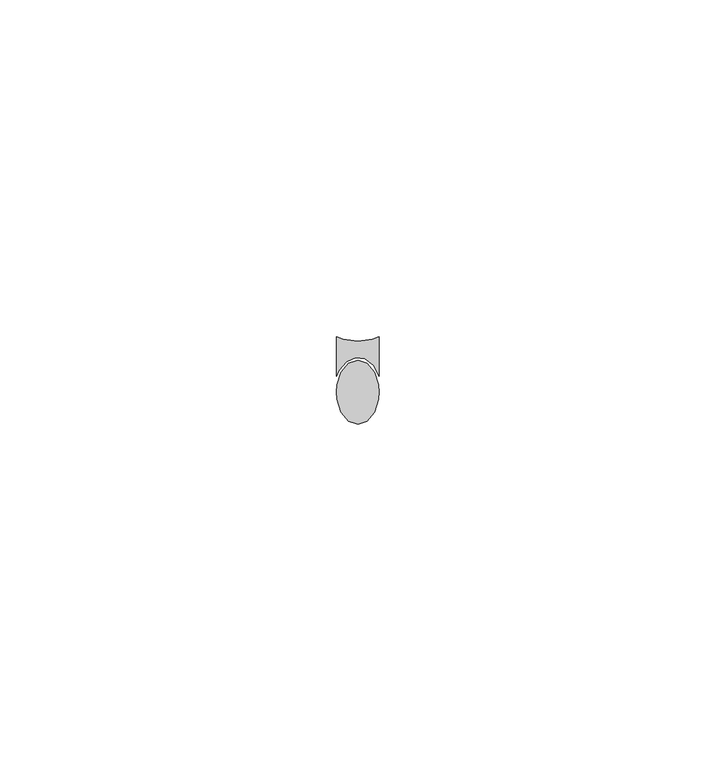
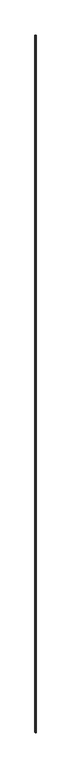
"""IFC4 building model written with IfcOpenShell, lengths in millimetres: proxy geometry, Generic Models 11:Generic Models 1:306267:Generic Models 1:306267 : Generic Models 11:Generic Models 1:306267:300405:Generic Models 1:306267:Generic Models 1:306267 : Generic Models 11:Generic Models 1:306267:300405 : Generic Models 11:Generic Models 1:306267:Generic Models 1:306267 : Generic Models 11:Generic Models 1:306267:300405:30 : Generic Models 11:Generic Models 1:306267:Generic Models 1:306267 : Generic Models 11:Generic Models 1:306267:300405:Generic Models 1:306267:Generic Models 1:306267 : Generic Models 11:Generic Models 1:306267:300405 : Generic Models 11:Generic Models 1:306267:Generic Models 1:306267 : Generic Models 11:Generic Models 1:306267:300405:300182."""

from ifc_helpers import new_model, si_unit, origin, origin_with_axes, place, context, project, spatial, polyline, outline, extrude, source, transform, mapped, element, save


def generic_models_00275e5b(model_context):
    return source(origin(), model_context, "Body", "SweptSolid", [
        extrude(outline(polyline([(593733.5341431, -556891.042805), (593734.9117239, -556890.5711692), (593736.2893048, -556891.042805), (593737.3940389, -556892.3642991), (593738.0071201, -556894.2739133), (593738.0867239, -556895.3336692), (593738.0071201, -556896.3934252), (593737.3940389, -556898.3030394), (593736.2893048, -556899.6245335), (593734.9117239, -556900.0961692), (593733.5341431, -556899.6245335), (593732.429409, -556898.3030394), (593731.8163278, -556896.3934252), (593731.7367239, -556895.3336692), (593731.8163278, -556894.2739133), (593732.429409, -556892.3642991), (593733.5341431, -556891.042805)])), origin_with_axes(), (0.0, 0.0, 1.0), 6064.4581746),
        extrude(outline(polyline([(593737.1209607, -556887.4793582), (593738.0867239, -556887.1019495), (593738.0867239, -556892.9700417), (593737.2039351, -556891.3768249), (593735.962551, -556890.4026199), (593734.5567747, -556890.199832), (593733.206527, -556890.8001855), (593732.1230415, -556892.1097607), (593731.7367239, -556892.9700417), (593731.7367239, -556887.1019495), (593732.7024872, -556887.4793582), (593734.9117239, -556887.7930442), (593737.1209607, -556887.4793582)])), origin_with_axes(), (0.0, 0.0, 1.0), 6062.9878028),
    ])


if __name__ == "__main__":
    model = new_model("IFC4")
    model_context = context("Model", 3, world=origin())
    ifc_project = project(units=[si_unit("LENGTHUNIT", "METRE", prefix="MILLI")], contexts=[model_context])
    site = spatial("IfcSite", under=ifc_project)
    building = spatial("IfcBuilding", under=site)
    placement = place(None, origin())
    generic_models_shape = generic_models_00275e5b(model_context)
    element("IfcBuildingElementProxy", 1, Name="Generic Models 11:Generic Models 1:306267:Generic Models 1:306267 : Generic Models 11:Generic Models 1:306267:300405:Generic Models 1:306267:Generic Models 1:306267 : Generic Models 11:Generic Models 1:306267:300405 : Generic Models 11:Generic Models 1:306267:Generic Models 1:306267 : Generic Models 11:Generic Models 1:306267:300405:30 : Generic Models 11:Generic Models 1:306267:Generic Models 1:306267 : Generic Models 11:Generic Models 1:306267:300405:Generic Models 1:306267:Generic Models 1:306267 : Generic Models 11:Generic Models 1:306267:300405 : Generic Models 11:Generic Models 1:306267:Generic Models 1:306267 : Generic Models 11:Generic Models 1:306267:300405:300182", ObjectType="Generic Models 11:Generic Models 1:306267:Generic Models 1:306267 : Generic Models 11:Generic Models 1:306267:300405:Generic Models 1:306267:Generic Models 1:306267 : Generic Models 11:Generic Models 1:306267:300405 : Generic Models 11:Generic Models 1:306267:Generic Models 1:306267 : Generic Models 11:Generic Models 1:306267:300405:30 : Generic Models 11:Generic Models 1:306267:Generic Models 1:306267 : Generic Models 11:Generic Models 1:306267:300405:Generic Models 1:306267:Generic Models 1:306267 : Generic Models 11:Generic Models 1:306267:300405 : Generic Models 11:Generic Models 1:306267:Generic Models 1:306267 : Generic Models 11:Generic Models 1:306267:300405:300182", at=placement, inside=building, context=model_context, shape_type="MappedRepresentation", body=[
        mapped(generic_models_shape, transform((0.0, 0.0, 0.0), x_axis=(1.0, 0.0, 0.0), y_axis=(0.0, 1.0, 0.0), z_axis=(0.0, 0.0, 1.0))),
    ])
    save(model, "model.ifc")

# Revit data of these elements
# Project information
#   IfcSite GUID = "2naYFwtnGHv906093rt3ko"
#   IfcBuilding GUID = "2naZIetnGHv906093rt3ko"
#   IfcProject GUID = "5efaeb93_8b82_4a45_8c7"
#   NumberOfStoreys = "1"
#   NameOverride = "Default"
#   Project Issue Date = "Issue Date"
#   Project Status = "Project Status"
#   Client Name = "Xcel"
#   Project Address = "Enter address here"
#   Project Name = "Sports Complex"
#   Project Number = "Project Number"
# Type "Generic Models 11:Generic Models 1:306267:Generic Models 1:306267 : Generic Models 11:Generic Models 1:306267:300405:Generic Models 1:306267:Generic Models 1:306267 : Generic Models 11:Generic Models 1:306267:300405 : Generic Models 11:Generic Models 1:306267:Generic Models 1:306267 : Generic Models 11:Generic Models 1:306267:300405:30 : Generic Models 11:Generic Models 1:306267:Generic Models 1:306267 : Generic Models 11:Generic Models 1:306267:300405:Generic Models 1:306267:Generic Models 1:306267 : Generic Models 11:Generic Models 1:306267:300405 : Generic Models 11:Generic Models 1:306267:Generic Models 1:306267 : Generic Models 11:Generic Models 1:306267:300405:300182"
#   NameOverride = "Generic Models 11:Generic Models 1:306267:Generic Models 1:306267 : Generic Models 11:Generic Models 1:306267:300405:Generic Models 1:306267:Generic Models 1:306267 : Generic Models 11:Generic Models 1:306267:300405 : Generic Models 11:Generic Models 1:306267:Generic Models 1:306267 : Generic Models 11:Generic Models 1:306267:300405:300182"
#   ObjectTypeOverride = "Generic Models 1:306267:Generic Models 1:306267 : Generic Models 11:Generic Models 1:306267:300405 : Generic Models 11:Generic Models 1:306267:Generic Models 1:306267 : Generic Models 11:Generic Models 1:306267:300405"
#   Reference = "Generic Models 1"
#   Tag = "300182"
# Element 1 (IfcBuildingElementProxy, "Generic Models 11:Generic Models 1:306267:Generic Models 1:306267 : Generic Models 11:Generic Models 1:306267:300405:Generic Models 1:306267:Generic Models 1:306267 : Generic Models 11:Generic Models 1:306267:300405 : Generic Models 11:Generic Models 1:306267:Generic Models 1:306267 : Generic Models 11:Generic Models 1:306267:300405:30 : Generic Models 11:Generic Models 1:306267:Generic Models 1:306267 : Generic Models 11:Generic Models 1:306267:300405:Generic Models 1:306267:Generic Models 1:306267 : Generic Models 11:Generic Models 1:306267:300405 : Generic Models 11:Generic Models 1:306267:Generic Models 1:306267 : Generic Models 11:Generic Models 1:306267:300405:300182")
#   Materials on its faces: "SEALANT & BACKER ROD, IF NECESSARY"
# Materials
#   "SEALANT & BACKER ROD, IF NECESSARY": class "Unassigned", colour RGB 120 120 120, transparency 0, Cost = 0
